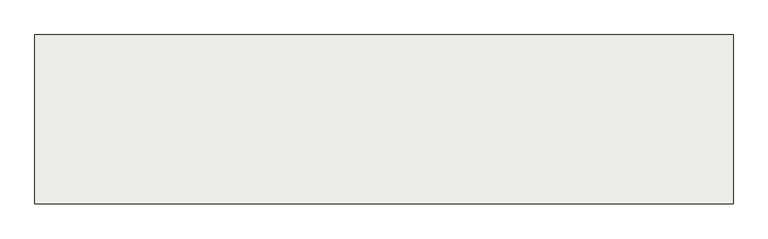
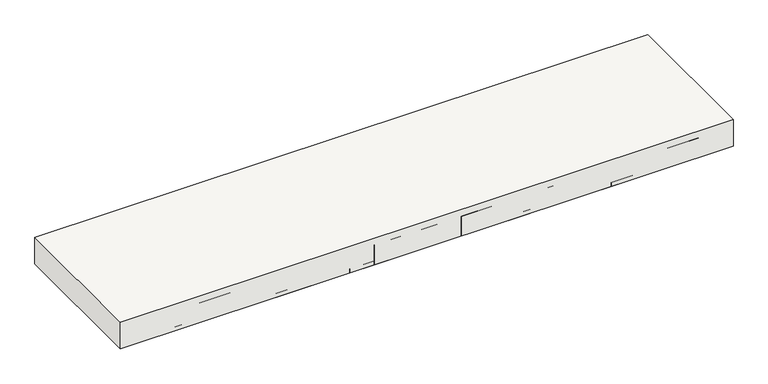
"""IFC4 building model written with IfcOpenShell, lengths in millimetres: slab geometry, Pano 15 (16 cm)."""

from ifc_helpers import new_model, si_unit, origin, origin_with_axes, place, context, project, spatial, polyline, outline, extrude, source, transform, mapped, element, save


def slab_267138a2(model_context):
    return source(origin(), model_context, "Body", "SweptSolid", [
        extrude(outline(polyline([(-860.0, 5350.0), (2655.0, 5350.0), (2655.0, 4500.0), (-860.0, 4500.0), (-860.0, 5350.0)])), origin_with_axes(), (0.0, 0.0, 1.0), 160.0),
        extrude(outline(polyline([(2455.0, 5000.0), (2095.0, 5000.0), (2095.0, 5345.0), (2455.0, 5345.0), (2455.0, 5000.0)])), origin_with_axes(), (0.0, 0.0, 1.0), 120.0),
        extrude(outline(polyline([(-45.0, 5000.0), (-405.0, 5000.0), (-405.0, 5345.0), (-45.0, 5345.0), (-45.0, 5000.0)])), origin_with_axes(), (0.0, 0.0, 1.0), 120.0),
        extrude(outline(polyline([(-45.0, 4500.0), (-405.0, 4500.0), (-405.0, 4995.0), (-45.0, 4995.0), (-45.0, 4500.0)])), origin_with_axes(), (0.0, 0.0, 1.0), 120.0),
        extrude(outline(polyline([(1955.0, 4500.0), (1595.0, 4500.0), (1595.0, 4995.0), (1955.0, 4995.0), (1955.0, 4500.0)])), origin_with_axes(), (0.0, 0.0, 1.0), 120.0),
        extrude(outline(polyline([(1595.0, 4500.0), (1455.0, 4500.0), (1455.0, 5350.0), (1595.0, 5350.0), (1595.0, 4500.0)])), origin_with_axes(), (0.0, 0.0, 1.0), 24.0),
        extrude(outline(polyline([(595.0, 4500.0), (455.0, 4500.0), (455.0, 5350.0), (595.0, 5350.0), (595.0, 4500.0)])), origin_with_axes(), (0.0, 0.0, 1.0), 24.0),
        extrude(outline(polyline([(1455.0, 4500.0), (1095.0, 4500.0), (1095.0, 4995.0), (1455.0, 4995.0), (1455.0, 4500.0)])), origin_with_axes(), (0.0, 0.0, 1.0), 120.0),
        extrude(outline(polyline([(1095.0, 4500.0), (955.0, 4500.0), (955.0, 5350.0), (1095.0, 5350.0), (1095.0, 4500.0)])), origin_with_axes(), (0.0, 0.0, 1.0), 24.0),
        extrude(outline(polyline([(2595.0, 4500.0), (2455.0, 4500.0), (2455.0, 5350.0), (2595.0, 5350.0), (2595.0, 4500.0)])), origin_with_axes(), (0.0, 0.0, 1.0), 24.0),
        extrude(outline(polyline([(2455.0, 4500.0), (2095.0, 4500.0), (2095.0, 4995.0), (2455.0, 4995.0), (2455.0, 4500.0)])), origin_with_axes(), (0.0, 0.0, 1.0), 120.0),
        extrude(outline(polyline([(455.0, 5000.0), (95.0, 5000.0), (95.0, 5345.0), (455.0, 5345.0), (455.0, 5000.0)])), origin_with_axes(), (0.0, 0.0, 1.0), 120.0),
        extrude(outline(polyline([(955.0, 5000.0), (595.0, 5000.0), (595.0, 5345.0), (955.0, 5345.0), (955.0, 5000.0)])), origin_with_axes(), (0.0, 0.0, 1.0), 120.0),
        extrude(outline(polyline([(95.0, 4500.0), (-45.0, 4500.0), (-45.0, 5350.0), (95.0, 5350.0), (95.0, 4500.0)])), origin_with_axes(), (0.0, 0.0, 1.0), 24.0),
        extrude(outline(polyline([(1455.0, 5000.0), (1095.0, 5000.0), (1095.0, 5345.0), (1455.0, 5345.0), (1455.0, 5000.0)])), origin_with_axes(), (0.0, 0.0, 1.0), 120.0),
        extrude(outline(polyline([(2095.0, 4500.0), (1955.0, 4500.0), (1955.0, 5350.0), (2095.0, 5350.0), (2095.0, 4500.0)])), origin_with_axes(), (0.0, 0.0, 1.0), 24.0),
        extrude(outline(polyline([(1955.0, 5000.0), (1595.0, 5000.0), (1595.0, 5345.0), (1955.0, 5345.0), (1955.0, 5000.0)])), origin_with_axes(), (0.0, 0.0, 1.0), 120.0),
        extrude(outline(polyline([(955.0, 4500.0), (595.0, 4500.0), (595.0, 4995.0), (955.0, 4995.0), (955.0, 4500.0)])), origin_with_axes(), (0.0, 0.0, 1.0), 120.0),
        extrude(outline(polyline([(455.0, 4500.0), (95.0, 4500.0), (95.0, 4995.0), (455.0, 4995.0), (455.0, 4500.0)])), origin_with_axes(), (0.0, 0.0, 1.0), 120.0),
        extrude(outline(polyline([(-405.0, 4500.0), (-545.0, 4500.0), (-545.0, 5350.0), (-405.0, 5350.0), (-405.0, 4500.0)])), origin_with_axes(), (0.0, 0.0, 1.0), 24.0),
    ])


if __name__ == "__main__":
    model = new_model("IFC4")
    model_context = context("Model", 3, world=origin())
    ifc_project = project(units=[si_unit("LENGTHUNIT", "METRE", prefix="MILLI")], contexts=[model_context])
    site = spatial("IfcSite", under=ifc_project)
    building = spatial("IfcBuilding", under=site)
    placement = place(None, origin())
    slab_shape = slab_267138a2(model_context)
    element("IfcSlab", 1, ObjectType="Pano 15 (16 cm)", at=placement, inside=building, context=model_context, shape_type="MappedRepresentation", body=[
        mapped(slab_shape, transform((0.0, 0.0, 0.0), x_axis=(1.0, 0.0, 0.0), y_axis=(0.0, 1.0, 0.0), z_axis=(0.0, 0.0, 1.0))),
    ])
    save(model, "model.ifc")

# Revit data of these elements
# Element 1 (IfcSlab, "Pano 15 (16 cm)")
#   Materials on its faces: "Molde de poliestireno", "Concreto armado", "RGB 168-169-158"
# Materials
#   "Molde de poliestireno": class "Não atribuído", colour RGB 255 255 255, transparency 0
#   "Concreto armado": class "Não atribuído", colour RGB 168 169 158, transparency 0
#   "RGB 168-169-158": class "Não atribuído", colour RGB 168 169 158, transparency 0
